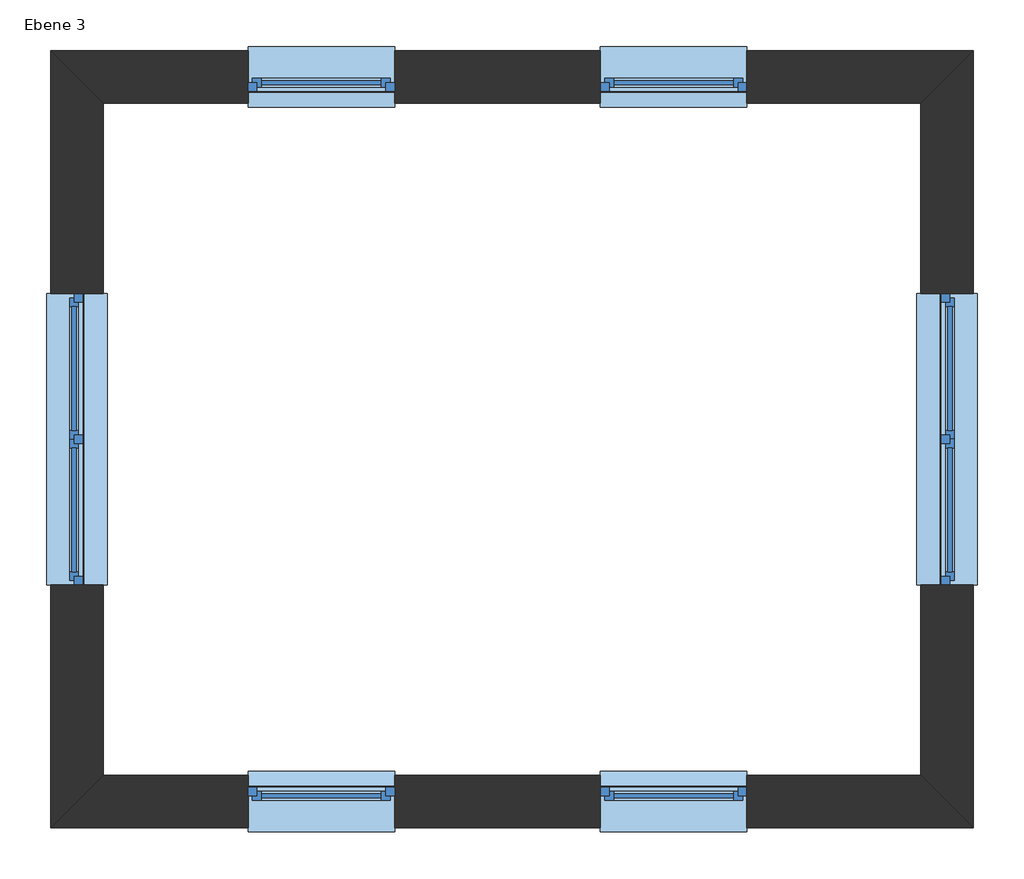
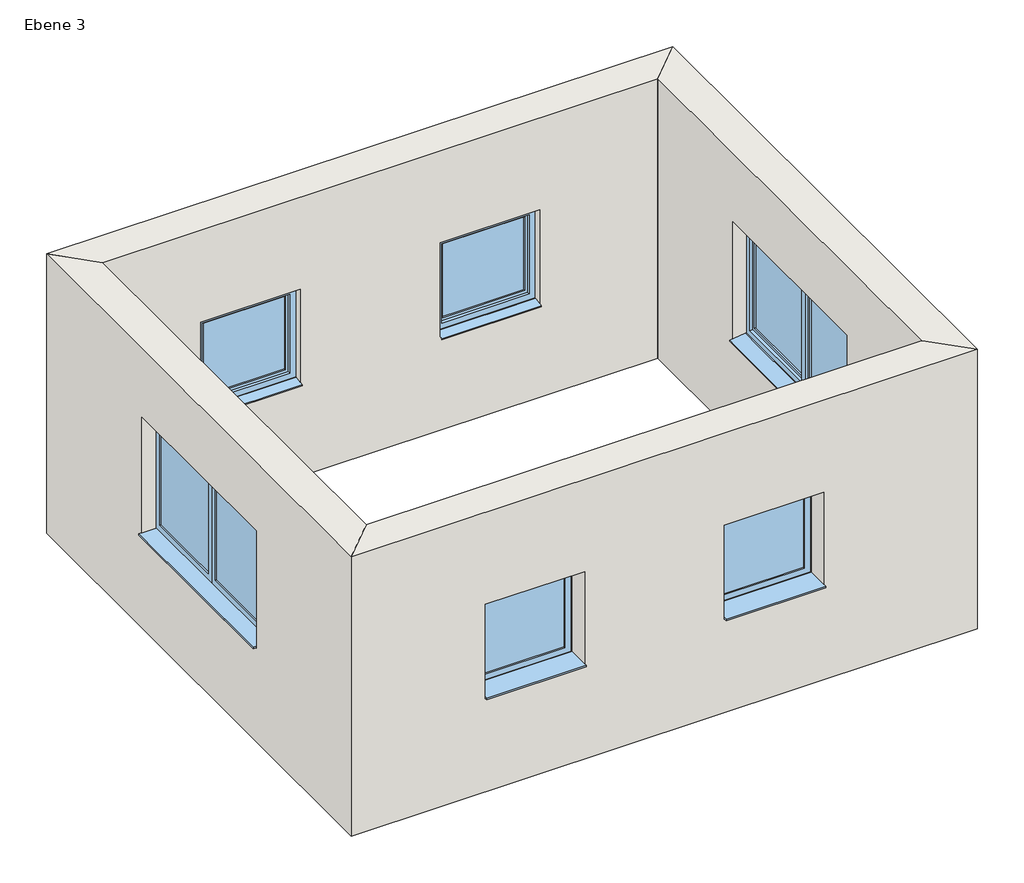
# One storey: 6 windows, 4 walls.
"""IFC4 building model written with IfcOpenShell, lengths in millimetres."""

import ifcopenshell
import ifcopenshell.guid

model = None  # the IFC model being written
_history = None  # IfcOwnerHistory: only IFC2X3 demands one
_inside = {}  # id of a spatial element -> (the spatial element, [elements in it])
_under = {}  # id of a project, library or spatial element -> (it, [spatial elements below it])
_declared = {}  # id of a project -> (the project, [libraries it declares])
_typed = {}  # id of a type object -> (the type object, [elements of that type])
_made_of = {}  # id of a material, layer set ... -> (it, [elements and type objects made of it])


def new_model(schema):
    """Start an empty IFC model of exactly this schema.

    Asked for "IFC4X3", IfcOpenShell would pick the latest addendum, in which some entities
    have other attributes; the version numbers below select the first issue.
    IFC2X3 requires an IfcOwnerHistory on every rooted entity: one is made here for all.
    """
    global model, _history
    if schema == "IFC4X3":
        model = ifcopenshell.file(schema_version=(4, 3, 0, 0))
    else:
        model = ifcopenshell.file(schema=schema)
    _inside.clear()
    _under.clear()
    _declared.clear()
    _typed.clear()
    _made_of.clear()
    _history = None
    if model.schema == "IFC2X3":
        org = make("IfcOrganization", Name="unknown")
        user = make(
            "IfcPersonAndOrganization",
            ThePerson=make("IfcPerson", FamilyName="unknown"),
            TheOrganization=org,
        )
        app = make(
            "IfcApplication",
            ApplicationDeveloper=org,
            Version="unknown",
            ApplicationFullName="unknown",
            ApplicationIdentifier="unknown",
        )
        _history = make(
            "IfcOwnerHistory",
            OwningUser=user,
            OwningApplication=app,
            ChangeAction="ADDED",
            CreationDate=0,
        )
    return model


def make(cls, **values):
    """One entity of the class cls with the attributes given. An attribute that is None is left unset."""
    return model.create_entity(
        cls, **{name: value for name, value in values.items() if value is not None}
    )


def rooted(cls, **values):
    """An entity with a GlobalId (a new one), such as an element, a storey or a relation."""
    return make(cls, GlobalId=ifcopenshell.guid.new(), OwnerHistory=_history, **values)


def si_unit(unit_type, name, prefix=None):
    """IfcSIUnit, for example si_unit("LENGTHUNIT", "METRE", prefix="MILLI")."""
    return make("IfcSIUnit", UnitType=unit_type, Prefix=prefix, Name=name)


def assignment(units):
    """IfcUnitAssignment: the units of a project."""
    return None if units is None else make("IfcUnitAssignment", Units=units)


def point(xyz):
    """IfcCartesianPoint."""
    return None if xyz is None else make("IfcCartesianPoint", Coordinates=xyz)


def direction(xyz):
    """IfcDirection."""
    return None if xyz is None else make("IfcDirection", DirectionRatios=xyz)


def frame(location, z_axis=None, x_axis=None):
    """IfcAxis2Placement3D, a coordinate frame: its origin and axes. An axis left out is left unset."""
    return make(
        "IfcAxis2Placement3D",
        Location=point(location),
        Axis=direction(z_axis),
        RefDirection=direction(x_axis),
    )


def origin():
    """The frame at (0, 0, 0) with its axes left unset."""
    return frame((0.0, 0.0, 0.0))


def place(relative_to, where):
    """IfcLocalPlacement: puts the frame where relative to a parent placement (None: the world)."""
    return make(
        "IfcLocalPlacement", PlacementRelTo=relative_to, RelativePlacement=where
    )


def context(
    kind, dimensions, precision=None, world=None, true_north=None, identifier=None
):
    """IfcGeometricRepresentationContext, for example the 3D "Model" context."""
    return make(
        "IfcGeometricRepresentationContext",
        ContextIdentifier=identifier,
        ContextType=kind,
        CoordinateSpaceDimension=dimensions,
        Precision=precision,
        WorldCoordinateSystem=world,
        TrueNorth=true_north,
    )


def project(units=None, contexts=None):
    """IfcProject with its units and contexts."""
    return rooted(
        "IfcProject",
        Name="project",
        RepresentationContexts=contexts,
        UnitsInContext=assignment(units),
    )


def spatial(cls, under=None, at=None, **own):
    """A site, building, storey or space (cls), placed at a placement, below another one or the project."""
    s = rooted(cls, ObjectPlacement=at, **own)
    if under is not None:
        _under.setdefault(under.id(), (under, []))[1].append(s)
    return s


def polyline(points):
    """IfcPolyline through the points."""
    return make("IfcPolyline", Points=[point(p) for p in points])


def outline(outer, holes=None, kind="AREA"):
    """IfcArbitraryClosedProfileDef: a profile drawn as a closed curve; with holes, ...WithVoids."""
    if holes is None:
        return make("IfcArbitraryClosedProfileDef", ProfileType=kind, OuterCurve=outer)
    return make(
        "IfcArbitraryProfileDefWithVoids",
        ProfileType=kind,
        OuterCurve=outer,
        InnerCurves=holes,
    )


def extrude(swept, where, along, depth):
    """IfcExtrudedAreaSolid: the profile swept, set in the frame where, extruded along a direction by depth."""
    return make(
        "IfcExtrudedAreaSolid",
        SweptArea=swept,
        Position=where,
        ExtrudedDirection=direction(along),
        Depth=depth,
    )


def faces_of(points, faces, orient=None, outer=None):
    """IfcFace entities. A face is a list of loops; a loop is a list of indices into points, from 0.

    orient and outer hold one flag for each loop. By default every Orientation is true, the
    first loop of a face is its IfcFaceOuterBound and the others are IfcFaceBound.
    """
    made = []
    for i, loops in enumerate(faces):
        bounds = []
        for j, loop in enumerate(loops):
            is_outer = j == 0 if outer is None else outer[i][j]
            bounds.append(
                make(
                    "IfcFaceOuterBound" if is_outer else "IfcFaceBound",
                    Bound=make("IfcPolyLoop", Polygon=[points[k] for k in loop]),
                    Orientation=True if orient is None else orient[i][j],
                )
            )
        made.append(make("IfcFace", Bounds=bounds))
    return made


def faceted_brep(points, faces, orient=None, outer=None, voids=None):
    """IfcFacetedBrep: a solid bounded by flat faces; with voids (closed shells), ...WithVoids."""
    shared = [point(p) for p in points]
    hull = make("IfcClosedShell", CfsFaces=faces_of(shared, faces, orient, outer))
    if voids is None:
        return make("IfcFacetedBrep", Outer=hull)
    return make(
        "IfcFacetedBrepWithVoids",
        Outer=hull,
        Voids=[
            make(cls, CfsFaces=faces_of(shared, fs, o, b)) for cls, fs, o, b in voids
        ],
    )


def shape(context_of_items, identifier, shape_type, items):
    """IfcShapeRepresentation: the items that make up one representation, for example the "Body"."""
    return make(
        "IfcShapeRepresentation",
        ContextOfItems=context_of_items,
        RepresentationIdentifier=identifier,
        RepresentationType=shape_type,
        Items=items,
    )


def source(mapping_origin, context_of_items, identifier, shape_type, items):
    """IfcRepresentationMap: a shape defined once, which mapped items show again and again."""
    return make(
        "IfcRepresentationMap",
        MappingOrigin=mapping_origin,
        MappedRepresentation=shape(context_of_items, identifier, shape_type, items),
    )


def transform(
    local_origin,
    x_axis=None,
    y_axis=None,
    z_axis=None,
    scale=None,
    scale2=None,
    scale3=None,
    uniform=True,
):
    """IfcCartesianTransformationOperator3D, or its non-uniform kind. x_axis, y_axis, z_axis: its Axis1, 2, 3."""
    if uniform:
        return make(
            "IfcCartesianTransformationOperator3D",
            Axis1=direction(x_axis),
            Axis2=direction(y_axis),
            LocalOrigin=point(local_origin),
            Scale=scale,
            Axis3=direction(z_axis),
        )
    return make(
        "IfcCartesianTransformationOperator3DnonUniform",
        Axis1=direction(x_axis),
        Axis2=direction(y_axis),
        LocalOrigin=point(local_origin),
        Scale=scale,
        Axis3=direction(z_axis),
        Scale2=scale2,
        Scale3=scale3,
    )


def mapped(mapping_source, mapping_target):
    """IfcMappedItem: shows the shape of a source again, moved by a transform."""
    return make(
        "IfcMappedItem", MappingSource=mapping_source, MappingTarget=mapping_target
    )


def made_of(thing, what):
    """Note that an element or type object is made of a material, layer set ...; save() writes the relation."""
    if what is not None:
        _made_of.setdefault(what.id(), (what, []))[1].append(thing)
    return thing


def element(
    cls,
    number,
    at=None,
    inside=None,
    cuts=None,
    type_object=None,
    material=None,
    context=None,
    identifier="Body",
    shape_type=None,
    held_by="IfcProductDefinitionShape",
    body=None,
    shapes=None,
    **own,
):
    """One element of the class cls, such as IfcWall. Its Tag is "e" and its number.

    at: its placement. inside: the storey or other place that contains it. cuts: it is an
    opening in that element (IfcRelVoidsElement). A single representation is given by context,
    identifier, shape_type and body (its items); several are given by shapes. held_by: the class
    of the entity that holds the representations. save() writes the other relations.
    """
    e = rooted(cls, Tag="e%d" % number, ObjectPlacement=at, **own)
    if body is not None:
        shapes = [shape(context, identifier, shape_type, body)]
    if shapes is not None:
        e.Representation = make(held_by, Representations=shapes)
    if inside is not None:
        _inside.setdefault(inside.id(), (inside, []))[1].append(e)
    if cuts is not None:
        rooted(
            "IfcRelVoidsElement", RelatingBuildingElement=cuts, RelatedOpeningElement=e
        )
    if type_object is not None:
        _typed.setdefault(type_object.id(), (type_object, []))[1].append(e)
    return made_of(e, material)


def aggregate(whole, parts):
    """IfcRelAggregates: a whole, such as a stair, and the parts it consists of."""
    return rooted("IfcRelAggregates", RelatingObject=whole, RelatedObjects=parts)


def save(model, path):
    """Write the relations noted so far, then the file.

    IfcRelAggregates (storeys below a building ...), IfcRelContainedInSpatialStructure (elements
    in a storey), IfcRelDefinesByType, IfcRelAssociatesMaterial and IfcRelDeclares: one each for
    every whole, place, type object, material and project.
    """
    for whole, parts in _under.values():
        aggregate(whole, parts)
    for where, things in _inside.values():
        rooted(
            "IfcRelContainedInSpatialStructure",
            RelatedElements=things,
            RelatingStructure=where,
        )
    for kind, things in _typed.values():
        rooted("IfcRelDefinesByType", RelatedObjects=things, RelatingType=kind)
    for what, things in _made_of.values():
        rooted("IfcRelAssociatesMaterial", RelatedObjects=things, RelatingMaterial=what)
    for by, libraries in _declared.values():
        rooted("IfcRelDeclares", RelatingContext=by, RelatedDefinitions=libraries)
    model.write(path)


def fenster_1_flg_variabel_fenster_1_flg_variabel_3_8a378bad(model_context):
    return source(origin(), model_context, "Body", "SolidModel", [
        extrude(outline(polyline([(2010.0, 505.0), (2010.0, -505.0), (1000.0, -505.0), (1000.0, 505.0), (2010.0, 505.0)]), holes=[polyline([(1930.0, 445.0), (1080.0, 445.0), (1080.0, -445.0), (1930.0, -445.0), (1930.0, 445.0)])]), frame((0.0, 40.0, 0.0), z_axis=(0.0, 1.0, 0.0), x_axis=(0.0, 0.0, 1.0)), (0.0, 0.0, 1.0), 60.0),
        faceted_brep([(475.0, 40.0, 1960.0), (475.0, 10.0, 1960.0), (475.0, 10.0, 1050.0), (475.0, 40.0, 1050.0), (-475.0, 10.0, 1960.0), (-475.0, 10.0, 1050.0), (415.0, 10.0, 1110.0), (-415.0, 10.0, 1110.0), (-415.0, 10.0, 1900.0), (415.0, 10.0, 1900.0), (-475.0, 40.0, 1050.0), (-475.0, 40.0, 1960.0), (445.0, 40.0, 1930.0), (-445.0, 40.0, 1930.0), (-445.0, 40.0, 1080.0), (445.0, 40.0, 1080.0), (445.0, 70.0, 1930.0), (445.0, 70.0, 1080.0), (-445.0, 70.0, 1080.0), (-445.0, 70.0, 1930.0), (415.0, 70.0, 1900.0), (-415.0, 70.0, 1900.0), (-415.0, 70.0, 1110.0), (415.0, 70.0, 1110.0)], [[[0, 1, 2, 3]], [[1, 4, 5, 2], [6, 7, 8, 9]], [[3, 2, 5, 10]], [[3, 10, 11, 0], [12, 13, 14, 15]], [[16, 12, 15, 17]], [[17, 15, 14, 18]], [[17, 18, 19, 16], [20, 21, 22, 23]], [[9, 20, 23, 6]], [[6, 23, 22, 7]], [[10, 5, 4, 11]], [[18, 14, 13, 19]], [[7, 22, 21, 8]], [[11, 4, 1, 0]], [[19, 13, 12, 16]], [[8, 21, 20, 9]]]),
        extrude(outline(polyline([(-505.0, -210.0), (-505.0, 40.0), (505.0, 40.0), (505.0, -210.0), (-505.0, -210.0)])), frame((0.0, 0.0, 1005.0), z_axis=(0.0, 0.0, 1.0), x_axis=(1.0, 0.0, 0.0)), (0.0, 0.0, 1.0), 15.0),
        extrude(outline(polyline([(110.0221543, 1020.0), (210.0, 1000.0), (210.0, 990.0), (208.0, 990.0), (208.0, 998.3604634), (109.8240723, 1018.0), (100.0, 1018.0), (100.0, 1020.0), (110.0221543, 1020.0)])), frame((-505.0, 0.0, 0.0), z_axis=(1.0, 0.0, 0.0), x_axis=(0.0, 1.0, 0.0)), (0.0, 0.0, 1.0), 1010.0),
        extrude(outline(polyline([(415.0, 25.0), (-415.0, 25.0), (-415.0, 55.0), (415.0, 55.0), (415.0, 25.0)])), frame((0.0, 0.0, 1110.0), z_axis=(0.0, 0.0, 1.0), x_axis=(1.0, 0.0, 0.0)), (0.0, 0.0, 1.0), 790.0),
    ])


def fenster_2_flg_variabel_fenster_2_flg_variabel_3_03287464(model_context):
    return source(origin(), model_context, "Body", "SolidModel", [
        extrude(outline(polyline([(60.0, -5.0), (915.0, -5.0), (915.0, -35.0), (60.0, -35.0), (60.0, -5.0)])), frame((0.0, 0.0, 1110.0), z_axis=(0.0, 0.0, 1.0), x_axis=(1.0, 0.0, 0.0)), (0.0, 0.0, 1.0), 1040.0),
        extrude(outline(polyline([(-915.0, -5.0), (-60.0, -5.0), (-60.0, -35.0), (-915.0, -35.0), (-915.0, -5.0)])), frame((0.0, 0.0, 1110.0), z_axis=(0.0, 0.0, 1.0), x_axis=(1.0, 0.0, 0.0)), (0.0, 0.0, 1.0), 1040.0),
        extrude(outline(polyline([(-1005.0, -210.0), (-1005.0, -20.0), (1005.0, -20.0), (1005.0, -210.0), (-1005.0, -210.0)])), frame((0.0, 0.0, 1005.0), z_axis=(0.0, 0.0, 1.0), x_axis=(1.0, 0.0, 0.0)), (0.0, 0.0, 1.0), 15.0),
        extrude(outline(polyline([(50.0221543, 1020.0), (210.0, 1000.0), (210.0, 990.0), (208.0, 990.0), (208.0, 998.3604634), (49.8240723, 1018.0), (40.0, 1018.0), (40.0, 1020.0), (50.0221543, 1020.0)])), frame((-1005.0, 0.0, 0.0), z_axis=(1.0, 0.0, 0.0), x_axis=(0.0, 1.0, 0.0)), (0.0, 0.0, 1.0), 2010.0),
        extrude(outline(polyline([(30.0, -20.0), (-30.0, -20.0), (-30.0, 40.0), (30.0, 40.0), (30.0, -20.0)])), frame((0.0, 0.0, 1080.0), z_axis=(0.0, 0.0, 1.0), x_axis=(1.0, 0.0, 0.0)), (0.0, 0.0, 1.0), 1100.0),
        extrude(outline(polyline([(2260.0, -1005.0), (1000.0, -1005.0), (1000.0, 1005.0), (2260.0, 1005.0), (2260.0, -1005.0)]), holes=[polyline([(2180.0, -945.0), (2180.0, 945.0), (1080.0, 945.0), (1080.0, -945.0), (2180.0, -945.0)])]), frame((0.0, -20.0, 0.0), z_axis=(0.0, 1.0, 0.0), x_axis=(0.0, 0.0, 1.0)), (0.0, 0.0, 1.0), 60.0),
        faceted_brep([(-945.0, -20.0, 1080.0), (-945.0, 10.0, 1080.0), (-30.0, 10.0, 1080.0), (-30.0, -20.0, 1080.0), (-30.0, 10.0, 2180.0), (-30.0, -20.0, 2180.0), (-945.0, 10.0, 2180.0), (-60.0, 10.0, 2150.0), (-915.0, 10.0, 2150.0), (-915.0, 10.0, 1110.0), (-60.0, 10.0, 1110.0), (0.0, -20.0, 1050.0), (-975.0, -20.0, 1050.0), (-975.0, -20.0, 2210.0), (0.0, -20.0, 2210.0), (-945.0, -20.0, 2180.0), (-975.0, -50.0, 1050.0), (0.0, -50.0, 1050.0), (0.0, -50.0, 2210.0), (-975.0, -50.0, 2210.0), (-60.0, -50.0, 1110.0), (-915.0, -50.0, 1110.0), (-915.0, -50.0, 2150.0), (-60.0, -50.0, 2150.0)], [[[0, 1, 2, 3]], [[3, 2, 4, 5]], [[2, 1, 6, 4], [7, 8, 9, 10]], [[11, 12, 13, 14], [5, 15, 0, 3]], [[16, 12, 11, 17]], [[17, 11, 14, 18]], [[18, 19, 16, 17], [20, 21, 22, 23]], [[9, 21, 20, 10]], [[10, 20, 23, 7]], [[15, 6, 1, 0]], [[19, 13, 12, 16]], [[8, 22, 21, 9]], [[5, 4, 6, 15]], [[18, 14, 13, 19]], [[7, 23, 22, 8]]]),
        faceted_brep([(30.0, -20.0, 1080.0), (30.0, 10.0, 1080.0), (945.0, 10.0, 1080.0), (945.0, -20.0, 1080.0), (945.0, 10.0, 2180.0), (945.0, -20.0, 2180.0), (30.0, 10.0, 2180.0), (915.0, 10.0, 2150.0), (60.0, 10.0, 2150.0), (60.0, 10.0, 1110.0), (915.0, 10.0, 1110.0), (975.0, -20.0, 1050.0), (0.0, -20.0, 1050.0), (0.0, -20.0, 2210.0), (975.0, -20.0, 2210.0), (30.0, -20.0, 2180.0), (0.0, -50.0, 1050.0), (975.0, -50.0, 1050.0), (975.0, -50.0, 2210.0), (0.0, -50.0, 2210.0), (915.0, -50.0, 1110.0), (60.0, -50.0, 1110.0), (60.0, -50.0, 2150.0), (915.0, -50.0, 2150.0)], [[[0, 1, 2, 3]], [[3, 2, 4, 5]], [[2, 1, 6, 4], [7, 8, 9, 10]], [[11, 12, 13, 14], [5, 15, 0, 3]], [[16, 12, 11, 17]], [[17, 11, 14, 18]], [[18, 19, 16, 17], [20, 21, 22, 23]], [[9, 21, 20, 10]], [[10, 20, 23, 7]], [[15, 6, 1, 0]], [[19, 13, 12, 16]], [[8, 22, 21, 9]], [[5, 4, 6, 15]], [[18, 14, 13, 19]], [[7, 23, 22, 8]]]),
    ])


model = new_model("IFC4")

# Units and contexts
model_context = context("Model", 3, world=origin())
ifc_project = project(units=[si_unit("LENGTHUNIT", "METRE", prefix="MILLI")], contexts=[model_context])

# Site, building, storey
site = spatial("IfcSite", under=ifc_project)
building = spatial("IfcBuilding", under=site)
storey = spatial("IfcBuildingStorey", under=building, Name="Ebene 3", Elevation=9000.0)

# Walls
placement = place(None, origin())
element("IfcWall", 1, ObjectType="MW 24.0 WD 12.0", at=placement, inside=storey, context=model_context, shape_type="Brep", body=[
    faceted_brep([(-6003.5987005, 5004.2257101, 9000.0), (-363.5987005, 5004.2257101, 9000.0), (-363.5987005, 5004.2257101, 12000.0), (-6003.5987005, 5004.2257101, 12000.0), (-1563.5987005, 5004.2257101, 10000.0), (-2573.5987005, 5004.2257101, 10000.0), (-2573.5987005, 5004.2257101, 11010.0), (-1563.5987005, 5004.2257101, 11010.0), (-3993.5987005, 5004.2257101, 10000.0), (-5003.5987005, 5004.2257101, 10000.0), (-5003.5987005, 5004.2257101, 11010.0), (-3993.5987005, 5004.2257101, 11010.0), (-6363.5987005, 5364.2257101, 9000.0), (-6363.5987005, 5364.2257101, 12000.0), (-3.5987005, 5364.2257101, 12000.0), (-3.5987005, 5364.2257101, 9000.0), (-1563.5987005, 5364.2257101, 10000.0), (-1563.5987005, 5364.2257101, 11010.0), (-2573.5987005, 5364.2257101, 11010.0), (-2573.5987005, 5364.2257101, 10000.0), (-3993.5987005, 5364.2257101, 10000.0), (-3993.5987005, 5364.2257101, 11010.0), (-5003.5987005, 5364.2257101, 11010.0), (-5003.5987005, 5364.2257101, 10000.0)], [[[0, 1, 2, 3], [4, 5, 6, 7], [8, 9, 10, 11]], [[12, 13, 14, 15], [16, 17, 18, 19], [20, 21, 22, 23]], [[1, 0, 12, 15]], [[3, 2, 14, 13]], [[2, 1, 15, 14]], [[0, 3, 13, 12]], [[17, 16, 4, 7]], [[18, 17, 7, 6]], [[19, 18, 6, 5]], [[16, 19, 5, 4]], [[21, 20, 8, 11]], [[22, 21, 11, 10]], [[23, 22, 10, 9]], [[20, 23, 9, 8]]]),
])
element("IfcWall", 2, ObjectType="MW 24.0 WD 12.0", at=placement, inside=storey, context=model_context, shape_type="Brep", body=[
    faceted_brep([(-363.5987005, 5004.2257101, 9000.0), (-363.5987005, 364.2257101, 9000.0), (-363.5987005, 364.2257101, 12000.0), (-363.5987005, 5004.2257101, 12000.0), (-363.5987005, 1679.2257101, 10000.0), (-363.5987005, 3689.2257101, 10000.0), (-363.5987005, 3689.2257101, 11260.0), (-363.5987005, 1679.2257101, 11260.0), (-3.5987005, 5364.2257101, 9000.0), (-3.5987005, 5364.2257101, 12000.0), (-3.5987005, 4.2257101, 12000.0), (-3.5987005, 4.2257101, 9000.0), (-3.5987005, 1679.2257101, 10000.0), (-3.5987005, 1679.2257101, 11260.0), (-3.5987005, 3689.2257101, 11260.0), (-3.5987005, 3689.2257101, 10000.0)], [[[0, 1, 2, 3], [4, 5, 6, 7]], [[8, 9, 10, 11], [12, 13, 14, 15]], [[1, 0, 8, 11]], [[3, 2, 10, 9]], [[0, 3, 9, 8]], [[2, 1, 11, 10]], [[13, 12, 4, 7]], [[14, 13, 7, 6]], [[15, 14, 6, 5]], [[12, 15, 5, 4]]]),
])
element("IfcWall", 3, ObjectType="MW 24.0 WD 12.0", at=placement, inside=storey, context=model_context, shape_type="Brep", body=[
    faceted_brep([(-363.5987005, 364.2257101, 9000.0), (-6003.5987005, 364.2257101, 9000.0), (-6003.5987005, 364.2257101, 12000.0), (-363.5987005, 364.2257101, 12000.0), (-2573.5987005, 364.2257101, 10000.0), (-1563.5987005, 364.2257101, 10000.0), (-1563.5987005, 364.2257101, 11010.0), (-2573.5987005, 364.2257101, 11010.0), (-5003.5987005, 364.2257101, 10000.0), (-3993.5987005, 364.2257101, 10000.0), (-3993.5987005, 364.2257101, 11010.0), (-5003.5987005, 364.2257101, 11010.0), (-3.5987005, 4.2257101, 9000.0), (-3.5987005, 4.2257101, 12000.0), (-6363.5987005, 4.2257101, 12000.0), (-6363.5987005, 4.2257101, 9000.0), (-2573.5987005, 4.2257101, 10000.0), (-2573.5987005, 4.2257101, 11010.0), (-1563.5987005, 4.2257101, 11010.0), (-1563.5987005, 4.2257101, 10000.0), (-5003.5987005, 4.2257101, 10000.0), (-5003.5987005, 4.2257101, 11010.0), (-3993.5987005, 4.2257101, 11010.0), (-3993.5987005, 4.2257101, 10000.0)], [[[0, 1, 2, 3], [4, 5, 6, 7], [8, 9, 10, 11]], [[12, 13, 14, 15], [16, 17, 18, 19], [20, 21, 22, 23]], [[1, 0, 12, 15]], [[3, 2, 14, 13]], [[0, 3, 13, 12]], [[2, 1, 15, 14]], [[17, 16, 4, 7]], [[18, 17, 7, 6]], [[19, 18, 6, 5]], [[16, 19, 5, 4]], [[21, 20, 8, 11]], [[22, 21, 11, 10]], [[23, 22, 10, 9]], [[20, 23, 9, 8]]]),
])
element("IfcWall", 4, ObjectType="MW 24.0 WD 12.0", at=placement, inside=storey, context=model_context, shape_type="Brep", body=[
    faceted_brep([(-6003.5987005, 364.2257101, 9000.0), (-6003.5987005, 5004.2257101, 9000.0), (-6003.5987005, 5004.2257101, 12000.0), (-6003.5987005, 364.2257101, 12000.0), (-6003.5987005, 3689.2257101, 10000.0), (-6003.5987005, 1679.2257101, 10000.0), (-6003.5987005, 1679.2257101, 11260.0), (-6003.5987005, 3689.2257101, 11260.0), (-6363.5987005, 4.2257101, 9000.0), (-6363.5987005, 4.2257101, 12000.0), (-6363.5987005, 5364.2257101, 12000.0), (-6363.5987005, 5364.2257101, 9000.0), (-6363.5987005, 3689.2257101, 10000.0), (-6363.5987005, 3689.2257101, 11260.0), (-6363.5987005, 1679.2257101, 11260.0), (-6363.5987005, 1679.2257101, 10000.0)], [[[0, 1, 2, 3], [4, 5, 6, 7]], [[8, 9, 10, 11], [12, 13, 14, 15]], [[1, 0, 8, 11]], [[3, 2, 10, 9]], [[2, 1, 11, 10]], [[0, 3, 9, 8]], [[13, 12, 4, 7]], [[14, 13, 7, 6]], [[15, 14, 6, 5]], [[12, 15, 5, 4]]]),
])

# Windows
fenster_1_flg_variabel_fenster_1_flg_variabel_3_shape = fenster_1_flg_variabel_fenster_1_flg_variabel_3_8a378bad(model_context)
element("IfcWindow", 5, ObjectType="Fenster 1-flg - Variabel : Fenster 1-flg - Variabel 3", at=placement, inside=storey, context=model_context, shape_type="MappedRepresentation", body=[
    mapped(fenster_1_flg_variabel_fenster_1_flg_variabel_3_shape, transform((-2068.5987005, 184.2257101, 9000.0), x_axis=(1.0, 0.0, 0.0), y_axis=(0.0, 1.0, 0.0), z_axis=(0.0, 0.0, 1.0))),
])
element("IfcWindow", 6, ObjectType="Fenster 1-flg - Variabel : Fenster 1-flg - Variabel 3", at=placement, inside=storey, context=model_context, shape_type="MappedRepresentation", body=[
    mapped(fenster_1_flg_variabel_fenster_1_flg_variabel_3_shape, transform((-4498.5987005, 184.2257101, 9000.0), x_axis=(1.0, 0.0, 0.0), y_axis=(0.0, 1.0, 0.0), z_axis=(0.0, 0.0, 1.0))),
])
element("IfcWindow", 7, ObjectType="Fenster 1-flg - Variabel : Fenster 1-flg - Variabel 3", at=placement, inside=storey, context=model_context, shape_type="MappedRepresentation", body=[
    mapped(fenster_1_flg_variabel_fenster_1_flg_variabel_3_shape, transform((-2068.5987005, 5184.2257101, 9000.0), x_axis=(-1.0, 0.0, 0.0), y_axis=(0.0, -1.0, 0.0), z_axis=(0.0, 0.0, 1.0))),
])
element("IfcWindow", 8, ObjectType="Fenster 1-flg - Variabel : Fenster 1-flg - Variabel 3", at=placement, inside=storey, context=model_context, shape_type="MappedRepresentation", body=[
    mapped(fenster_1_flg_variabel_fenster_1_flg_variabel_3_shape, transform((-4498.5987005, 5184.2257101, 9000.0), x_axis=(-1.0, 0.0, 0.0), y_axis=(0.0, -1.0, 0.0), z_axis=(0.0, 0.0, 1.0))),
])
fenster_2_flg_variabel_fenster_2_flg_variabel_3_shape = fenster_2_flg_variabel_fenster_2_flg_variabel_3_03287464(model_context)
element("IfcWindow", 9, ObjectType="Fenster 2-flg - Variabel : Fenster 2-flg - Variabel 3", at=placement, inside=storey, context=model_context, shape_type="MappedRepresentation", body=[
    mapped(fenster_2_flg_variabel_fenster_2_flg_variabel_3_shape, transform((-183.5987005, 2684.2257101, 9000.0), x_axis=(0.0, 1.0, 0.0), y_axis=(-1.0, 0.0, 0.0), z_axis=(0.0, 0.0, 1.0))),
])
element("IfcWindow", 10, ObjectType="Fenster 2-flg - Variabel : Fenster 2-flg - Variabel 3", at=placement, inside=storey, context=model_context, shape_type="MappedRepresentation", body=[
    mapped(fenster_2_flg_variabel_fenster_2_flg_variabel_3_shape, transform((-6183.5987005, 2684.2257101, 9000.0), x_axis=(0.0, -1.0, 0.0), y_axis=(1.0, 0.0, 0.0), z_axis=(0.0, 0.0, 1.0))),
])

save(model, "model.ifc")

# Revit data of these elements
# Type "MW 24.0 WD 12.0"
#   Type Comments = "Mehrschaliges Mauerwerk"
#   Description = "Mauerwerk 24.0 cm, Wärmedämmung 12.0 cm"
#   Layers, outside or top first: 0.120 m "Wärmedämmung - hart" (function 3); 0.240 m "Mauerwerk - Ziegel, verputzt" (function 1)
# Type "Fenster 1-flg - Variabel : Fenster 1-flg - Variabel 3"
#   Type Mark = "52"
#   Operation = "SinglePanel"
#   Construction Type Id = "GSP4R"
#   Keynote = "16.05.01"
#   Analytic Construction = "1/8 Zoll Pilkington-Verglasung einfach"
#   Cost = 78.2
#   Visual Light Transmittance = 0.9
#   Höhe oberer  Rahmen = 0.080 m
#   Solar Heat Gain Coefficient = 0.86
#   Tiefe Flügel = 0.060 m
#   Rough Width [instance default] = 1.010 m
#   Rough Height [instance default] = 1.010 m
#   Rahmenhöhe unten = 0.080 m
#   Heat Transfer Coefficient (U) = 6.7069 W/(m²·K)
#   Rahmentiefe = 0.060 m
#   Rahmenbreite = 0.060 m
#   Height [instance default] = 1.010 m
#   Flügelbreite = 0.060 m
#   Einbautiefe (von außen) [instance default] = 0.080 m
#   Width [instance default] = 1.010 m
#   Define Thermal Properties by = 1
#   Öffnungsrichtung oben [instance default] = yes
#   Öffnungsrichtung in Draufsicht anzeigen [instance default] = no
#   Klappflügel [instance default] = no
#   Drehflügel 1 [instance default] = yes
#   Fensterflügel [instance default] = none
#   Innere Fensterbank [instance default] = none
#   Glas [instance default] = none
#   Bild [instance default] = none
#   Äußere Fensterbank [instance default] = none
#   Wall Closure = (empty or 0)
# Type "Fenster 2-flg - Variabel : Fenster 2-flg - Variabel 3"
#   Type Mark = "53"
#   Operation = "DoublePanelVertical"
#   Construction Type Id = "GSP4R"
#   Keynote = "16.05.01"
#   Analytic Construction = "1/8 Zoll Pilkington-Verglasung einfach"
#   Cost = 130.98
#   Visual Light Transmittance = 0.9
#   Solar Heat Gain Coefficient = 0.78
#   Rough Width [instance default] = 2.010 m
#   Rough Height [instance default] = 1.260 m
#   Heat Transfer Coefficient (U) = 3.6886 W/(m²·K)
#   Rahmentiefe = 0.060 m
#   Rahmenhöhe unten = 0.080 m
#   Höhe oberer  Rahmen = 0.080 m
#   Rahmenbreite = 0.060 m
#   Height [instance default] = 1.260 m
#   Tiefe Flügel = 0.060 m
#   Flügelbreite = 0.060 m
#   Einbautiefe (von außen) [instance default] = 0.140 m
#   Width [instance default] = 2.010 m
#   Define Thermal Properties by = 1
#   Öffnungsrichtung oben [instance default] = yes
#   Öffnungsrichtung in Draufsicht anzeigen [instance default] = no
#   Drehflügel 1 [instance default] = yes
#   Bild [instance default] = none
#   Glas [instance default] = none
#   Fensterflügel [instance default] = none
#   Äußere Fensterbank [instance default] = none
#   Innere Fensterbank [instance default] = none
#   Wall Closure = (empty or 0)
# Elements 1, 2, 3, 4 (IfcWall, "MW 24.0 WD 12.0")
#   Comments = ""
#   Top Offset = 0.000 m
#   Base Offset = 0.000 m
#   Unconnected Height = 3.000 m
#   wall height = 3.000 m
#   Phase Created = Phase 1
#   Base Constraint = Ebene 3
#   Materials on its faces: "Vorgabe - Wand", "Mauerwerk - Ziegel, verputzt", "Wärmedämmung - hart"
# Element 5 (IfcWindow, "Fenster 1-flg - Variabel : Fenster 1-flg - Variabel 3")
#   Mark = "16"
#   Rough Height = 1.010 m
#   Rough Width = 1.010 m
#   Height = 1.010 m
#   Einbautiefe (von außen) = 0.080 m
#   Width = 1.010 m
#   Öffnungsrichtung oben = yes
#   Öffnungsrichtung in Draufsicht anzeigen = no
#   Klappflügel = no
#   Drehflügel 1 = yes
#   Äußere Fensterbank = none
#   Innere Fensterbank = none
#   Glas = none
#   Fensterflügel = none
#   Bild = none
#   Phase Created = Phase 1
#   Materials on its faces: "Kunststoff - Weiß", "Holz - Birke", "Glas"
# Element 6 (IfcWindow, "Fenster 1-flg - Variabel : Fenster 1-flg - Variabel 3")
#   Mark = "17"
#   Rough Height = 1.010 m
#   Rough Width = 1.010 m
#   Height = 1.010 m
#   Einbautiefe (von außen) = 0.080 m
#   Width = 1.010 m
#   Öffnungsrichtung oben = yes
#   Öffnungsrichtung in Draufsicht anzeigen = no
#   Klappflügel = no
#   Drehflügel 1 = yes
#   Äußere Fensterbank = none
#   Innere Fensterbank = none
#   Glas = none
#   Fensterflügel = none
#   Bild = none
#   Phase Created = Phase 1
#   Materials on its faces: "Kunststoff - Weiß", "Holz - Birke", "Glas"
# Element 7 (IfcWindow, "Fenster 1-flg - Variabel : Fenster 1-flg - Variabel 3")
#   Mark = "18"
#   Rough Height = 1.010 m
#   Rough Width = 1.010 m
#   Height = 1.010 m
#   Einbautiefe (von außen) = 0.080 m
#   Width = 1.010 m
#   Öffnungsrichtung oben = yes
#   Öffnungsrichtung in Draufsicht anzeigen = no
#   Klappflügel = no
#   Drehflügel 1 = yes
#   Äußere Fensterbank = none
#   Innere Fensterbank = none
#   Glas = none
#   Fensterflügel = none
#   Bild = none
#   Phase Created = Phase 1
#   Materials on its faces: "Kunststoff - Weiß", "Holz - Birke", "Glas"
# Element 8 (IfcWindow, "Fenster 1-flg - Variabel : Fenster 1-flg - Variabel 3")
#   Mark = "19"
#   Rough Height = 1.010 m
#   Rough Width = 1.010 m
#   Height = 1.010 m
#   Einbautiefe (von außen) = 0.080 m
#   Width = 1.010 m
#   Öffnungsrichtung oben = yes
#   Öffnungsrichtung in Draufsicht anzeigen = no
#   Klappflügel = no
#   Drehflügel 1 = yes
#   Äußere Fensterbank = none
#   Innere Fensterbank = none
#   Glas = none
#   Fensterflügel = none
#   Bild = none
#   Phase Created = Phase 1
#   Materials on its faces: "Kunststoff - Weiß", "Holz - Birke", "Glas"
# Element 9 (IfcWindow, "Fenster 2-flg - Variabel : Fenster 2-flg - Variabel 3")
#   Mark = "20"
#   Rough Height = 1.260 m
#   Rough Width = 2.010 m
#   Height = 1.260 m
#   Einbautiefe (von außen) = 0.140 m
#   Width = 2.010 m
#   Öffnungsrichtung oben = yes
#   Öffnungsrichtung in Draufsicht anzeigen = no
#   Drehflügel 1 = yes
#   Äußere Fensterbank = none
#   Innere Fensterbank = none
#   Glas = none
#   Fensterflügel = none
#   Bild = none
#   Phase Created = Phase 1
#   Materials on its faces: "Kunststoff - Weiß", "Glas", "Holz - Birke"
# Element 10 (IfcWindow, "Fenster 2-flg - Variabel : Fenster 2-flg - Variabel 3")
#   Mark = "21"
#   Rough Height = 1.260 m
#   Rough Width = 2.010 m
#   Height = 1.260 m
#   Einbautiefe (von außen) = 0.140 m
#   Width = 2.010 m
#   Öffnungsrichtung oben = yes
#   Öffnungsrichtung in Draufsicht anzeigen = no
#   Drehflügel 1 = yes
#   Äußere Fensterbank = none
#   Innere Fensterbank = none
#   Glas = none
#   Fensterflügel = none
#   Bild = none
#   Phase Created = Phase 1
#   Materials on its faces: "Kunststoff - Weiß", "Glas", "Holz - Birke"
# Materials
#   "Wärmedämmung - hart": class "Stuck", colour RGB 255 255 255, transparency 0, Description = "Äußere Oberfläche", Cost = 0
#   "Mauerwerk - Ziegel, verputzt": class "Stuck", colour RGB 247 247 247, transparency 0, Cost = 0
#   "Vorgabe - Wand": class "Stuck", colour RGB 128 128 128, transparency 0, Description = "Äußere Oberfläche", Cost = 0
#   "Kunststoff - Weiß": class "Kunststoff", colour RGB 249 249 249, transparency 0, Cost = 0
#   "Holz - Birke": class "Holz", colour RGB 213 164 103, transparency 0, Cost = 0
#   "Glas": class "Glas", colour RGB 0 0 255, transparency 0.75, Comments = "Render-Darstellung nicht aktualisiert ", Cost = 0
